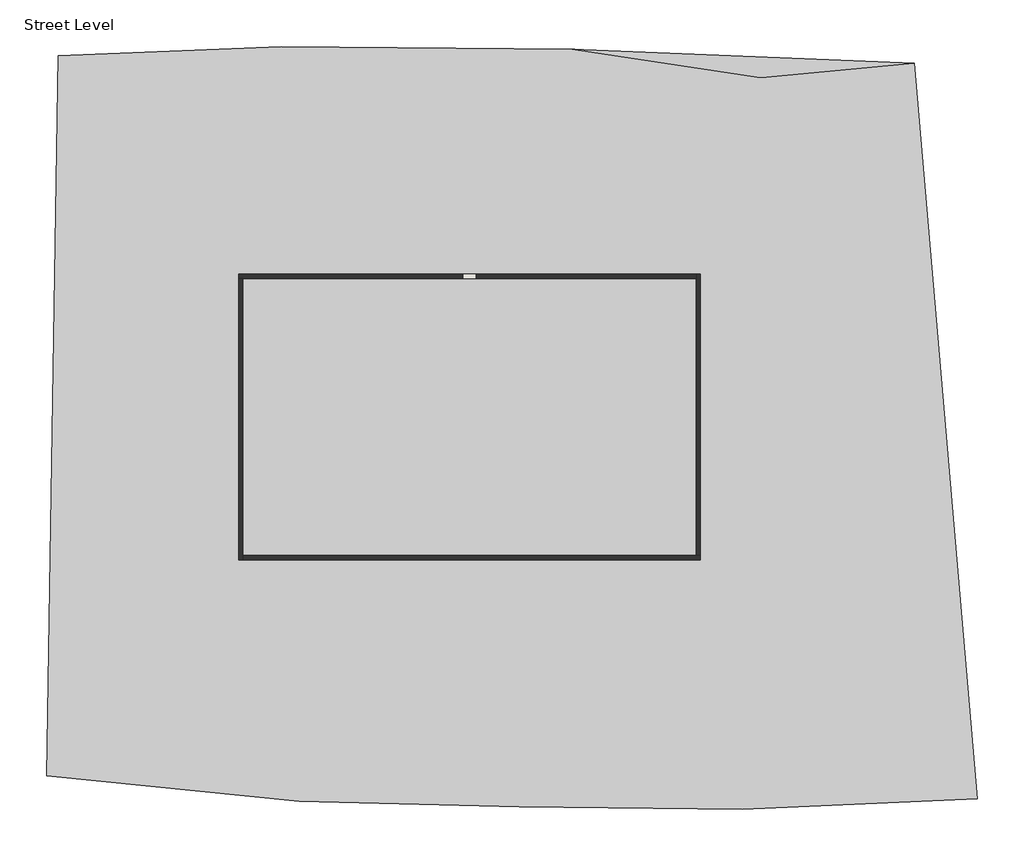
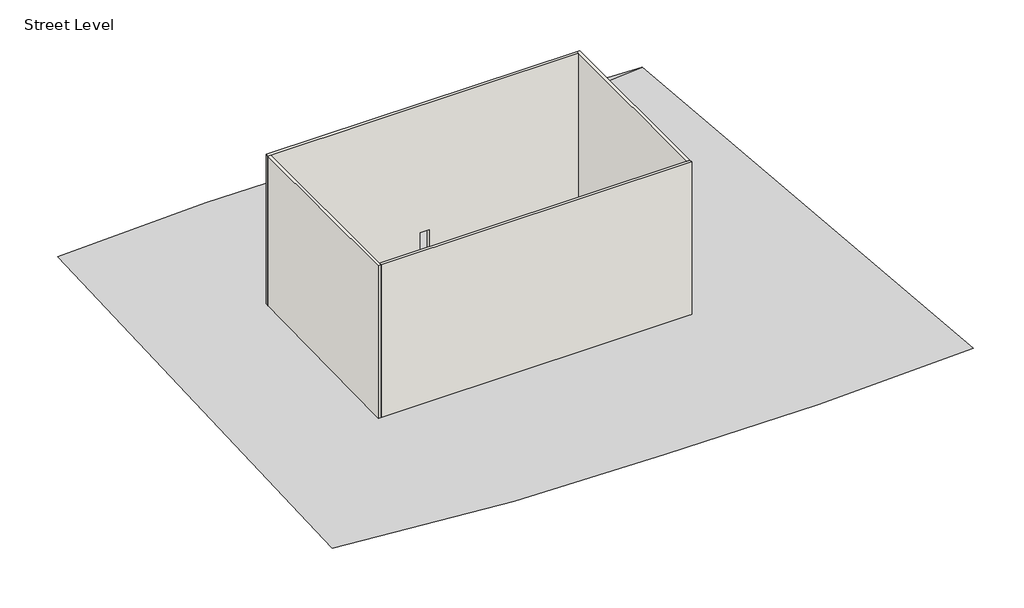
# One storey: 4 walls, 1 proxy.
"""IFC4 building model written with IfcOpenShell, lengths in millimetres."""

from ifc_helpers import new_model, si_unit, origin, place, context, project, spatial, faceted_brep, triangles, element, save

model = new_model("IFC4")

# Units and contexts
model_context = context("Model", 3, world=origin())
ifc_project = project(units=[si_unit("LENGTHUNIT", "METRE", prefix="MILLI")], contexts=[model_context])

# Site, building, storey
site = spatial("IfcSite", under=ifc_project)
building = spatial("IfcBuilding", under=site)
storey = spatial("IfcBuildingStorey", under=building, Name="Street Level", Elevation=-914.4)

# Proxy
placement = place(None, origin())
element("IfcBuildingElementProxy", 1, Name="Building Element Proxy", at=placement, inside=storey, context=model_context, shape_type="Tessellation", body=[
    triangles([(-29664.1428223, 25063.2445862, 0.0), (-14195.9393097, 25689.5644958, 0.0), (5935.7725708, 25510.6149536, 0.0), (18999.0170654, 23542.1816162, 0.0), (29646.4555298, 24526.3982849, 0.0), (-30469.4122742, -24863.4009705, -914.4), (-12943.2994904, -26652.8870911, -914.4), (2267.3273026, -27010.7838501, -914.4), (17746.3772461, -27189.7333923, -914.4), (34030.6948975, -26473.9375488, -914.4)], [[7, 8, 2], [6, 2, 1], [2, 6, 7], [8, 3, 2], [9, 10, 4], [3, 4, 5], [3, 8, 4], [5, 4, 10], [4, 8, 9]], closed=False),
])

# Walls
element("IfcWall", 2, ObjectType="Generic - 12\"", at=placement, inside=storey, context=model_context, shape_type="Brep", body=[
    faceted_brep([(-17167.8122732, 9596.3015304, -914.4), (-16863.0122732, 9596.3015304, -914.4), (14531.3877268, 9596.3015304, -914.4), (14531.3877268, 9596.3015304, 15849.6), (-16863.0122732, 9596.3015304, 15849.6), (-17167.8122732, 9596.3015304, 15849.6), (-708.6122732, 9596.3015304, 0.0), (-1623.0122732, 9596.3015304, 0.0), (-1623.0122732, 9596.3015304, 2133.6), (-708.6122732, 9596.3015304, 2133.6), (-17167.8122732, 9901.1015304, -914.4), (-17167.8122732, 9901.1015304, 15849.6), (14531.3877268, 9901.1015304, 15849.6), (14531.3877268, 9901.1015304, -914.4), (-708.6122732, 9901.1015304, 0.0), (-708.6122732, 9901.1015304, 2133.6), (-1623.0122732, 9901.1015304, 2133.6), (-1623.0122732, 9901.1015304, 0.0)], [[[0, 1, 2, 3, 4, 5], [6, 7, 8, 9]], [[10, 11, 12, 13], [14, 15, 16, 17]], [[2, 1, 0, 10, 13]], [[5, 4, 3, 12, 11]], [[0, 5, 11, 10]], [[3, 2, 13, 12]], [[7, 6, 14, 17]], [[8, 7, 17, 16]], [[9, 8, 16, 15]], [[6, 9, 15, 14]]]),
])
element("IfcWall", 3, ObjectType="Generic - 12\"", at=placement, inside=storey, context=model_context, shape_type="Brep", body=[
    faceted_brep([(-16863.0122732, -9910.8984696, -914.4), (-16863.0122732, -9606.0984696, -914.4), (-16863.0122732, 9596.3015304, -914.4), (-16863.0122732, 9596.3015304, 15849.6), (-16863.0122732, -9606.0984696, 15849.6), (-16863.0122732, -9910.8984696, 15849.6), (-17167.8122732, -9910.8984696, -914.4), (-17167.8122732, -9910.8984696, 15849.6), (-17167.8122732, 9596.3015304, 15849.6), (-17167.8122732, 9596.3015304, -914.4)], [[[0, 1, 2, 3, 4, 5]], [[6, 7, 8, 9]], [[2, 1, 0, 6, 9]], [[5, 4, 3, 8, 7]], [[0, 5, 7, 6]], [[3, 2, 9, 8]]]),
])
element("IfcWall", 4, ObjectType="Generic - 12\"", at=placement, inside=storey, context=model_context, shape_type="Brep", body=[
    faceted_brep([(14836.1877268, -9606.0984696, -914.4), (14531.3877268, -9606.0984696, -914.4), (-16863.0122732, -9606.0984696, -914.4), (-16863.0122732, -9606.0984696, 15849.6), (14531.3877268, -9606.0984696, 15849.6), (14836.1877268, -9606.0984696, 15849.6), (14836.1877268, -9910.8984696, -914.4), (14836.1877268, -9910.8984696, 15849.6), (-16863.0122732, -9910.8984696, 15849.6), (-16863.0122732, -9910.8984696, -914.4)], [[[0, 1, 2, 3, 4, 5]], [[6, 7, 8, 9]], [[2, 1, 0, 6, 9]], [[5, 4, 3, 8, 7]], [[0, 5, 7, 6]], [[3, 2, 9, 8]]]),
])
element("IfcWall", 5, ObjectType="Generic - 12\"", at=placement, inside=storey, context=model_context, shape_type="Brep", body=[
    faceted_brep([(14531.3877268, 9901.1015304, -914.4), (14531.3877268, 9596.3015304, -914.4), (14531.3877268, -9606.0984696, -914.4), (14531.3877268, -9606.0984696, 15849.6), (14531.3877268, 9596.3015304, 15849.6), (14531.3877268, 9901.1015304, 15849.6), (14836.1877268, 9901.1015304, -914.4), (14836.1877268, 9901.1015304, 15849.6), (14836.1877268, -9606.0984696, 15849.6), (14836.1877268, -9606.0984696, -914.4)], [[[0, 1, 2, 3, 4, 5]], [[6, 7, 8, 9]], [[2, 1, 0, 6, 9]], [[5, 4, 3, 8, 7]], [[0, 5, 7, 6]], [[3, 2, 9, 8]]]),
])

save(model, "model.ifc")

# Revit data of these elements
# Project information
#   Organization Name = "G3B Press"
#   Organization Description = "Paul F. Aubin Cosulting Services, Inc."
#   Building Name = "Revit Essentials for Architecture"
#   Author = "Paul F. Aubin"
#   Author Website = "https://www.paulaubin.com"
#   Copyright = "Copyright © 2020 Paul F Aubin, all rights reserved"
#   Project Issue Date = "8/1/2020"
#   Project Status = "Design Development"
#   Client Name = "Setting Up Project Levels and Views"
#   Project Address = "123 State ST\nSuite 301\nChicago, IL 60606"
#   Project Name = "05 Commercial_Complete"
#   Project Number = "2020.04A"
# Type "Generic - 12\""
#   Assembly Code = "B2010"
#   Layers, outside or top first: 1' - 0" no material (function 1)
# Element 1 (IfcBuildingElementProxy)
#   Material = none
#   Phase Created = New Construction
# Elements 2, 3, 4, 5 (IfcWall, "Generic - 12\"")
#   Top Offset = 4' - 0"
#   Base Offset = 0' - 0"
#   wall height = 55' - 0"
#   Phase Created = New Construction
#   Base Constraint = Street Level
#   Top Constraint = Roof
#   Materials on its faces: "Default Wall"
# Materials
#   "Default Wall": class "Miscellaneous", colour RGB 128 128 128, transparency 0, Cost = 0
